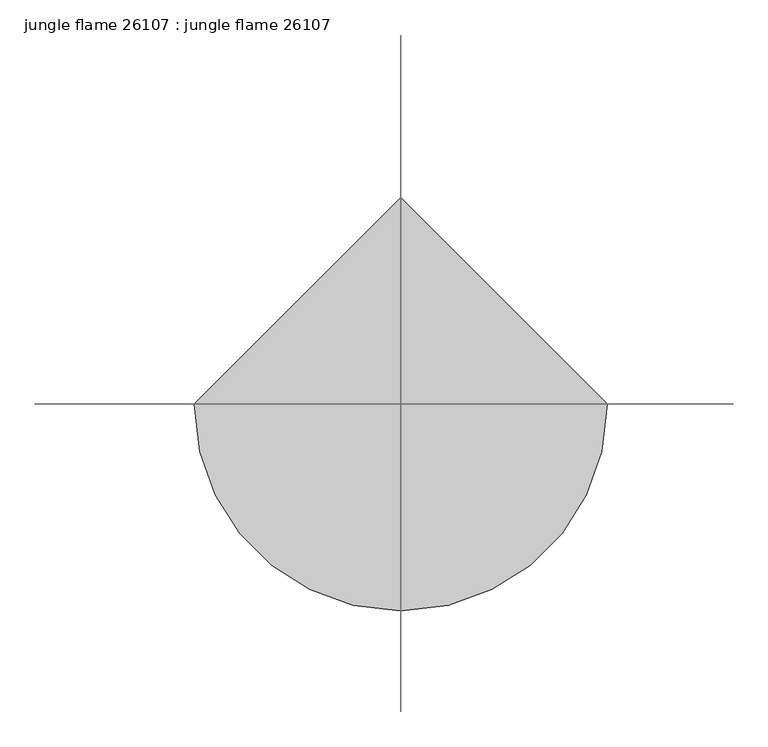
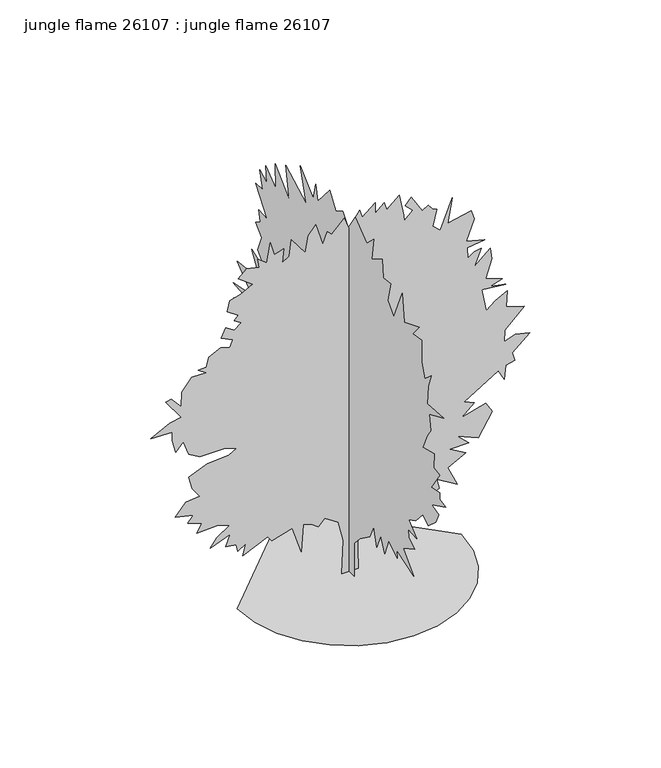
"""IFC4 building model written with IfcOpenShell, lengths in millimetres: proxy geometry, jungle flame 26107 : jungle flame 26107."""

import ifcopenshell
import ifcopenshell.guid

model = None  # the IFC model being written
_history = None  # IfcOwnerHistory: only IFC2X3 demands one
_inside = {}  # id of a spatial element -> (the spatial element, [elements in it])
_under = {}  # id of a project, library or spatial element -> (it, [spatial elements below it])
_declared = {}  # id of a project -> (the project, [libraries it declares])
_typed = {}  # id of a type object -> (the type object, [elements of that type])
_made_of = {}  # id of a material, layer set ... -> (it, [elements and type objects made of it])


def new_model(schema):
    """Start an empty IFC model of exactly this schema.

    Asked for "IFC4X3", IfcOpenShell would pick the latest addendum, in which some entities
    have other attributes; the version numbers below select the first issue.
    IFC2X3 requires an IfcOwnerHistory on every rooted entity: one is made here for all.
    """
    global model, _history
    if schema == "IFC4X3":
        model = ifcopenshell.file(schema_version=(4, 3, 0, 0))
    else:
        model = ifcopenshell.file(schema=schema)
    _inside.clear()
    _under.clear()
    _declared.clear()
    _typed.clear()
    _made_of.clear()
    _history = None
    if model.schema == "IFC2X3":
        org = make("IfcOrganization", Name="unknown")
        user = make(
            "IfcPersonAndOrganization",
            ThePerson=make("IfcPerson", FamilyName="unknown"),
            TheOrganization=org,
        )
        app = make(
            "IfcApplication",
            ApplicationDeveloper=org,
            Version="unknown",
            ApplicationFullName="unknown",
            ApplicationIdentifier="unknown",
        )
        _history = make(
            "IfcOwnerHistory",
            OwningUser=user,
            OwningApplication=app,
            ChangeAction="ADDED",
            CreationDate=0,
        )
    return model


def make(cls, **values):
    """One entity of the class cls with the attributes given. An attribute that is None is left unset."""
    return model.create_entity(
        cls, **{name: value for name, value in values.items() if value is not None}
    )


def rooted(cls, **values):
    """An entity with a GlobalId (a new one), such as an element, a storey or a relation."""
    return make(cls, GlobalId=ifcopenshell.guid.new(), OwnerHistory=_history, **values)


def si_unit(unit_type, name, prefix=None):
    """IfcSIUnit, for example si_unit("LENGTHUNIT", "METRE", prefix="MILLI")."""
    return make("IfcSIUnit", UnitType=unit_type, Prefix=prefix, Name=name)


def assignment(units):
    """IfcUnitAssignment: the units of a project."""
    return None if units is None else make("IfcUnitAssignment", Units=units)


def point(xyz):
    """IfcCartesianPoint."""
    return None if xyz is None else make("IfcCartesianPoint", Coordinates=xyz)


def direction(xyz):
    """IfcDirection."""
    return None if xyz is None else make("IfcDirection", DirectionRatios=xyz)


def frame(location, z_axis=None, x_axis=None):
    """IfcAxis2Placement3D, a coordinate frame: its origin and axes. An axis left out is left unset."""
    return make(
        "IfcAxis2Placement3D",
        Location=point(location),
        Axis=direction(z_axis),
        RefDirection=direction(x_axis),
    )


def origin():
    """The frame at (0, 0, 0) with its axes left unset."""
    return frame((0.0, 0.0, 0.0))


def place(relative_to, where):
    """IfcLocalPlacement: puts the frame where relative to a parent placement (None: the world)."""
    return make(
        "IfcLocalPlacement", PlacementRelTo=relative_to, RelativePlacement=where
    )


def context(
    kind, dimensions, precision=None, world=None, true_north=None, identifier=None
):
    """IfcGeometricRepresentationContext, for example the 3D "Model" context."""
    return make(
        "IfcGeometricRepresentationContext",
        ContextIdentifier=identifier,
        ContextType=kind,
        CoordinateSpaceDimension=dimensions,
        Precision=precision,
        WorldCoordinateSystem=world,
        TrueNorth=true_north,
    )


def project(units=None, contexts=None):
    """IfcProject with its units and contexts."""
    return rooted(
        "IfcProject",
        Name="project",
        RepresentationContexts=contexts,
        UnitsInContext=assignment(units),
    )


def spatial(cls, under=None, at=None, **own):
    """A site, building, storey or space (cls), placed at a placement, below another one or the project."""
    s = rooted(cls, ObjectPlacement=at, **own)
    if under is not None:
        _under.setdefault(under.id(), (under, []))[1].append(s)
    return s


def point_list(points):
    """IfcCartesianPointList2D or 3D."""
    cls = (
        "IfcCartesianPointList2D" if len(points[0]) == 2 else "IfcCartesianPointList3D"
    )
    return make(cls, CoordList=points)


def triangles(points, corners, closed=None, point_numbers=None):
    """IfcTriangulatedFaceSet: each triangle names its three corners, points numbered from 1."""
    return make(
        "IfcTriangulatedFaceSet",
        Coordinates=point_list(points),
        Closed=closed,
        CoordIndex=corners,
        PnIndex=point_numbers,
    )


def shape(context_of_items, identifier, shape_type, items):
    """IfcShapeRepresentation: the items that make up one representation, for example the "Body"."""
    return make(
        "IfcShapeRepresentation",
        ContextOfItems=context_of_items,
        RepresentationIdentifier=identifier,
        RepresentationType=shape_type,
        Items=items,
    )


def source(mapping_origin, context_of_items, identifier, shape_type, items):
    """IfcRepresentationMap: a shape defined once, which mapped items show again and again."""
    return make(
        "IfcRepresentationMap",
        MappingOrigin=mapping_origin,
        MappedRepresentation=shape(context_of_items, identifier, shape_type, items),
    )


def transform(
    local_origin,
    x_axis=None,
    y_axis=None,
    z_axis=None,
    scale=None,
    scale2=None,
    scale3=None,
    uniform=True,
):
    """IfcCartesianTransformationOperator3D, or its non-uniform kind. x_axis, y_axis, z_axis: its Axis1, 2, 3."""
    if uniform:
        return make(
            "IfcCartesianTransformationOperator3D",
            Axis1=direction(x_axis),
            Axis2=direction(y_axis),
            LocalOrigin=point(local_origin),
            Scale=scale,
            Axis3=direction(z_axis),
        )
    return make(
        "IfcCartesianTransformationOperator3DnonUniform",
        Axis1=direction(x_axis),
        Axis2=direction(y_axis),
        LocalOrigin=point(local_origin),
        Scale=scale,
        Axis3=direction(z_axis),
        Scale2=scale2,
        Scale3=scale3,
    )


def mapped(mapping_source, mapping_target):
    """IfcMappedItem: shows the shape of a source again, moved by a transform."""
    return make(
        "IfcMappedItem", MappingSource=mapping_source, MappingTarget=mapping_target
    )


def made_of(thing, what):
    """Note that an element or type object is made of a material, layer set ...; save() writes the relation."""
    if what is not None:
        _made_of.setdefault(what.id(), (what, []))[1].append(thing)
    return thing


def element(
    cls,
    number,
    at=None,
    inside=None,
    cuts=None,
    type_object=None,
    material=None,
    context=None,
    identifier="Body",
    shape_type=None,
    held_by="IfcProductDefinitionShape",
    body=None,
    shapes=None,
    **own,
):
    """One element of the class cls, such as IfcWall. Its Tag is "e" and its number.

    at: its placement. inside: the storey or other place that contains it. cuts: it is an
    opening in that element (IfcRelVoidsElement). A single representation is given by context,
    identifier, shape_type and body (its items); several are given by shapes. held_by: the class
    of the entity that holds the representations. save() writes the other relations.
    """
    e = rooted(cls, Tag="e%d" % number, ObjectPlacement=at, **own)
    if body is not None:
        shapes = [shape(context, identifier, shape_type, body)]
    if shapes is not None:
        e.Representation = make(held_by, Representations=shapes)
    if inside is not None:
        _inside.setdefault(inside.id(), (inside, []))[1].append(e)
    if cuts is not None:
        rooted(
            "IfcRelVoidsElement", RelatingBuildingElement=cuts, RelatedOpeningElement=e
        )
    if type_object is not None:
        _typed.setdefault(type_object.id(), (type_object, []))[1].append(e)
    return made_of(e, material)


def aggregate(whole, parts):
    """IfcRelAggregates: a whole, such as a stair, and the parts it consists of."""
    return rooted("IfcRelAggregates", RelatingObject=whole, RelatedObjects=parts)


def save(model, path):
    """Write the relations noted so far, then the file.

    IfcRelAggregates (storeys below a building ...), IfcRelContainedInSpatialStructure (elements
    in a storey), IfcRelDefinesByType, IfcRelAssociatesMaterial and IfcRelDeclares: one each for
    every whole, place, type object, material and project.
    """
    for whole, parts in _under.values():
        aggregate(whole, parts)
    for where, things in _inside.values():
        rooted(
            "IfcRelContainedInSpatialStructure",
            RelatedElements=things,
            RelatingStructure=where,
        )
    for kind, things in _typed.values():
        rooted("IfcRelDefinesByType", RelatedObjects=things, RelatingType=kind)
    for what, things in _made_of.values():
        rooted("IfcRelAssociatesMaterial", RelatedObjects=things, RelatingMaterial=what)
    for by, libraries in _declared.values():
        rooted("IfcRelDeclares", RelatingContext=by, RelatedDefinitions=libraries)
    model.write(path)


def jungle_flame_26107_jungle_flame_26107_31e44138(model_context):
    return source(origin(), model_context, "Body", "Tessellation", [
        triangles([(-297.8835799, 0.0, 5.16e-05), (-290.0095692, -68.2551316, 5.16e-05), (-267.5813779, -130.9367389, 5.16e-05), (-232.3950082, -186.2485517, 5.16e-05), (-186.2485517, -232.3952625, 5.16e-05), (-130.9367389, -267.5813779, 5.16e-05), (-68.2551316, -290.0095692, 5.16e-05), (1.3e-05, -297.8835799, 5.16e-05), (68.2551316, -290.0095692, 5.16e-05), (130.9367389, -267.5813779, 5.16e-05), (186.2485517, -232.3950082, 5.16e-05), (232.3952625, -186.2485517, 5.16e-05), (267.5813779, -130.9367389, 5.16e-05), (290.0095692, -68.2551316, 5.16e-05), (297.8835799, 2.6e-05, 5.16e-05), (-3.91e-05, 297.8835799, 5.16e-05), (-1.65e-05, -22.3446072, 4.98e-05), (-1.37e-05, -22.4089451, 93.4481205), (-1.4e-05, -48.2564431, 121.2837307), (-1.51e-05, -93.9863508, 155.0842657), (-1.48e-05, -113.868958, 194.849244), (-1.69e-05, -127.7866314, 145.1429666), (-1.64e-05, -145.6809334, 188.8845644), (-1.84e-05, -163.5752263, 149.1193318), (-1.77e-05, -181.4695374, 196.8375492), (-2.03e-05, -221.2347519, 170.9902534), (-1.95e-05, -219.2464467, 192.8611749), (-2.38e-05, -296.7888247, 167.0136247), (-2.02e-05, -249.070353, 216.7201655), (-2.16e-05, -300.7639273, 244.5557666), (-1.99e-05, -272.9306153, 260.4617543), (-1.92e-05, -270.9418014, 282.3336933), (-2.1e-05, -310.7054898, 280.3448793), (-1.85e-05, -274.9168858, 312.1558373), (-1.94e-05, -306.7304054, 328.0638416), (-1.98e-05, -338.5413634, 363.8524638), (-2.13e-05, -364.3884049, 349.9332553), (-2.2e-05, -398.1907022, 379.7579247), (-2.17e-05, -412.1073672, 409.5800869), (-2e-05, -380.2964092, 417.5353426), (-2.19e-05, -443.9208687, 449.3463006), (-2.05e-05, -416.0849951, 455.3102171), (-2e-05, -416.0849951, 473.2045464), (-1.85e-05, -378.3075771, 465.2517978), (-1.85e-05, -416.0849951, 522.9123407), (-1.71e-05, -388.2491578, 526.8874251), (-1.6e-05, -390.2379536, 566.6536752), (-1.41e-05, -338.5413634, 554.7232987), (-1.37e-05, -358.4244884, 598.4646332), (-1.37e-05, -374.3299493, 622.325386), (-1.22e-05, -368.3660328, 664.0779247), (-1.42e-05, -433.9793243, 693.9025578), (-1.1e-05, -358.4244884, 687.9386776), (-9.7e-06, -364.3884049, 741.6215927), (-9.1e-06, -376.3187814, 777.4101786), (-8.6e-06, -346.4940757, 751.5605936), (-6.8e-06, -332.5774469, 789.3380116), (-5e-06, -332.5774469, 850.9736389), (-3.4e-06, -292.8111969, 845.0096861), (-3.7e-06, -322.6358663, 880.7983446), (-1.4e-06, -253.0469816, 852.962471), (1.3e-06, -243.1056735, 928.5173069), (3e-07, -205.3287642, 839.0458059), (2.5e-06, -177.4931631, 868.8679682), (3.5e-06, -191.4108456, 924.5396427), (4.9e-06, -157.6105468, 920.564522), (6.6e-06, -151.6456129, 968.2810135), (7.9e-06, -103.9276498, 940.4451399), (9.3e-06, -111.8806437, 1000.0944786), (9.9e-06, -80.0684139, 970.2698456), (1.34e-05, -28.3738313, 1012.0223116), (1.33e-05, 3.4383978, 962.3170607), (1.55e-05, 29.285692, 994.128055), (1.63e-05, 61.0979195, 976.2337257), (1.88e-05, 88.9335251, 1015.9999758), (1.94e-05, 144.6047364, 952.3755163), (2.1e-05, 154.5460354, 994.128055), (2.02e-05, 166.475667, 946.4115635), (2.45e-05, 226.1232435, 1002.0833107), (2.06e-05, 198.2876424, 912.6118097), (2.63e-05, 291.7367712, 964.3058928), (2.3e-05, 275.8287488, 876.8232239), (2.77e-05, 339.4532264, 938.4588512), (2.56e-05, 337.4669377, 870.8567276), (2.87e-05, 383.1945608, 906.6453861), (2.71e-05, 379.2194401, 860.9151833), (2.91e-05, 411.0303981, 878.8095125), (2.7e-05, 397.113733, 831.0930937), (2.85e-05, 430.9135231, 829.1042616), (2.4e-05, 377.2306443, 759.5158493), (2.58e-05, 415.0080623, 763.49097), (2.47e-05, 409.0441458, 733.6662643), (2.52e-05, 430.9135231, 719.7495993), (2.32e-05, 403.0776858, 691.9137983), (2.26e-05, 420.9719788, 648.1724276), (1.97e-05, 381.2082722, 608.4061775), (2.34e-05, 448.807816, 632.2669304), (1.9e-05, 401.0888537, 554.7232987), (2.1e-05, 436.8774396, 568.6424709), (2.42e-05, 514.4211076, 558.7009266), (1.96e-05, 448.807816, 505.0180115), (2.28e-05, 532.3154005, 487.1237185), (1.85e-05, 440.8551038, 479.1710063), (1.74e-05, 430.9135231, 457.2990492), (2.16e-05, 530.3266047, 447.3575048), (1.66e-05, 438.8662717, 419.5216312), (1.6e-05, 456.7605646, 369.8163803), (1.51e-05, 409.0441458, 411.5688827), (1.33e-05, 395.1249372, 371.8051761), (1.47e-05, 442.8438995, 349.9332553), (1.34e-05, 444.8327316, 302.2142748), (9.7e-06, 379.2194401, 276.3672333), (1.12e-05, 426.9384387, 254.4978378), (5.4e-06, 323.5477292, 216.7201655), (7.3e-06, 379.2194401, 194.849244), (7.4e-06, 411.0303981, 151.1076461), (4.7e-06, 327.5253571, 184.9081902), (2.9e-06, 321.5588971, 135.2016584), (2.6e-06, 287.7591252, 174.966882), (0.0, 265.8897297, 119.2956707), (1.8e-06, 267.8760183, 176.9549329), (1.3e-06, 253.9588446, 182.9198668), (-1.2e-06, 226.1232435, 141.1663379), (-2e-07, 228.1115487, 170.9902534), (-2.1e-06, 180.3933313, 176.9549329), (-2.7e-06, 186.3580108, 151.1076461), (-3.4e-06, 154.5460354, 174.966882), (-6.1e-06, 144.6047364, 99.4130544), (-6.1e-06, 82.9688456, 190.8728697), (-7.1e-06, 69.0509133, 178.9432563), (-8.2e-06, 41.2153077, 182.9198668), (-8.5e-06, 57.1215497, 149.1193318), (-9.5e-06, 17.3562001, 174.966882), (-1.44e-05, 25.309295, 5.13e-05), (-19.2607679, 5.89e-05, 1.9e-06), (-15.3064967, 5.32e-05, 92.9241154), (-29.1462451, 5.05e-05, 148.2829094), (-64.7341846, 5.06e-05, 172.0082871), (-82.5281566, 5.25e-05, 154.2143151), (-100.3221195, 5.24e-05, 168.0540227), (-122.0703651, 5.3e-05, 173.9854194), (-128.0015165, 5.76e-05, 100.8324082), (-151.7268943, 5.43e-05, 173.9854194), (-205.1088103, 5.76e-05, 158.1685977), (-216.9713675, 5.72e-05, 173.9854194), (-282.2168581, 6.19e-05, 142.351758), (-274.3072937, 5.97e-05, 173.9854194), (-296.0547671, 6.15e-05, 160.14573), (-300.0095584, 6.05e-05, 179.9165799), (-327.6904633, 6.14e-05, 183.8708443), (-315.8261438, 5.9e-05, 215.5045239), (-369.2092953, 6.27e-05, 193.7565236), (-351.4140879, 6.05e-05, 217.4816561), (-317.8048021, 5.76e-05, 241.2070248), (-351.4140879, 5.85e-05, 251.0924498), (-404.7972393, 6.09e-05, 249.1153175), (-390.956805, 5.9e-05, 270.8630453), (-428.5208639, 5.98e-05, 284.7035159), (-414.6829368, 5.82e-05, 302.4962162), (-462.1326568, 5.95e-05, 314.3605356), (-434.4542953, 5.64e-05, 345.9937065), (-396.887693, 5.46e-05, 349.9484797), (-416.6590516, 5.38e-05, 377.6268774), (-426.5447127, 5.21e-05, 413.2148214), (-377.1163344, 4.86e-05, 434.9622949), (-319.780917, 4.59e-05, 438.917068), (-298.0334254, 4.42e-05, 450.7814238), (-333.6213876, 4.52e-05, 460.6645414), (-396.887693, 4.8e-05, 460.6645414), (-426.5447127, 4.82e-05, 478.4597852), (-440.3851833, 4.64e-05, 518.0025023), (-460.1565419, 4.86e-05, 496.2524855), (-470.0396959, 4.69e-05, 531.8404295), (-470.0396959, 4.55e-05, 555.5665612), (-527.3776568, 4.79e-05, 557.5426761), (-475.9731274, 4.41e-05, 583.2475024), (-446.3160713, 4.25e-05, 589.1783904), (-487.8349397, 4.09e-05, 646.5138079), (-472.0183542, 4e-05, 648.4899227), (-446.3160713, 4.07e-05, 618.8354101), (-444.337413, 3.82e-05, 658.3755838), (-418.6351665, 3.51e-05, 691.987413), (-379.0949927, 3.35e-05, 690.0087547), (-400.8424662, 3.35e-05, 705.8278473), (-379.0949927, 3.26e-05, 705.8278473), (-373.1615613, 3.08e-05, 731.5301302), (-341.5283904, 2.84e-05, 747.346752), (-317.8048021, 2.79e-05, 739.437133), (-309.8952195, 2.64e-05, 759.2085279), (-339.5522756, 2.68e-05, 773.0489622), (-327.6904633, 2.48e-05, 798.7512451), (-305.9404464, 2.47e-05, 784.9108109), (-286.1690878, 2.3e-05, 798.7512451), (-305.9404464, 2.31e-05, 810.6130211), (-294.0786522, 2.19e-05, 822.4748697), (-323.7356901, 2.2e-05, 842.246192), (-317.8048021, 2e-05, 871.903248), (-288.1477461, 1.82e-05, 879.8127943), (-256.5145934, 1.59e-05, 895.6293434), (-294.0786522, 1.58e-05, 925.2863995), (-272.3311788, 1.36e-05, 945.0577944), (-238.719604, 1.26e-05, 937.1482481), (-242.6736322, 1.14e-05, 960.8743435), (-218.9484997, 1.14e-05, 943.0791361), (-209.0628204, 7.8e-06, 996.4622875), (-199.1773955, 9.6e-06, 958.8956852), (-173.4748764, 8e-06, 966.8052315), (-177.429159, 1.04e-05, 929.2386292), (-159.635187, 8.9e-06, 941.1030212), (-153.7037722, 6.1e-06, 984.5979681), (-116.1389593, 7.4e-06, 935.1721333), (-108.2304123, 4.3e-06, 980.6457384), (-88.459308, 2.1e-06, 1004.3692904), (-70.6655904, 4.9e-06, 943.0791361), (-58.8027788, 2.5e-06, 974.712307), (-46.9402171, 2.7e-06, 962.8504583), (-13.329386, -7e-07, 996.4622875), (-1.4667204, 6e-07, 964.8265732), (28.1899354, -3e-06, 1004.3692904), (34.1210891, -2e-06, 982.6218533), (69.7090263, -5.2e-06, 1010.300251), (69.7090263, -3.4e-06, 980.6457384), (93.4344041, -5.8e-06, 1002.3931755), (99.3655555, -4.7e-06, 980.6457384), (132.9763673, -8e-06, 1010.300251), (144.8391788, -4.8e-06, 949.0100241), (146.816311, -4e-06, 933.1934023), (168.5642931, -6.2e-06, 954.9434555), (148.793198, -6.5e-06, 974.712307), (164.610283, -8.3e-06, 992.5075144), (194.2668122, -6.8e-06, 945.0577944), (210.083652, -8e-06, 954.9434555), (219.969077, -7.6e-06, 941.1030212), (231.8318885, -7.8e-06, 935.1721333), (221.9462092, -4.8e-06, 891.6745703), (241.7173134, -4.6e-06, 873.8819063), (273.3497213, -1.07e-05, 952.9647972), (261.487909, -6.2e-06, 885.7436823), (324.756776, -9.8e-06, 899.5841892), (332.6637789, -8.6e-06, 873.8819063), (310.9163054, -4.3e-06, 818.5225674), (360.3447201, -5.7e-06, 804.6821331), (312.8924203, -3.2e-06, 798.7512451), (314.8710786, -1.5e-06, 769.0941891), (332.6637789, -3e-06, 780.9560377), (350.4590226, -4e-06, 784.9108109), (332.6637789, -6e-07, 739.437133), (374.1826472, -4.6e-06, 777.0037354), (378.1374204, -2.9e-06, 745.3680937), (362.3208349, 7e-07, 695.9421862), (405.8183252, -2e-07, 680.1256371), (374.1826472, 1.8e-06, 670.2399759), (415.7014792, 5e-07, 660.3542421), (352.4351375, 2.8e-06, 668.2613176), (364.2969498, 6.1e-06, 604.9949759), (388.0230815, 3.9e-06, 624.7662981), (419.6562524, 1.5e-06, 640.5829199), (417.6801375, 4.2e-06, 597.0853932), (465.1298575, 3.1e-06, 581.2688441), (413.7253644, 8.3e-06, 531.8404295), (411.7492132, 1.02e-05, 500.2072586), (441.4037258, 8.2e-06, 512.0716144), (478.9703281, 7.2e-06, 502.1859169), (433.496723, 1.15e-05, 462.6431997), (439.427611, 1.27e-05, 438.917068), (415.7014792, 1.41e-05, 432.98618), (411.7492132, 1.65e-05, 395.4221211), (395.9326641, 1.54e-05, 425.0765974), (304.9854175, 2.27e-05, 369.7198382), (332.6637789, 2.22e-05, 357.8555188), (297.075853, 2.55e-05, 328.1984628), (362.3208349, 2.16e-05, 345.9937065), (380.1135352, 2.26e-05, 316.3366868), (342.5494763, 2.79e-05, 255.046478), (287.1901737, 2.89e-05, 278.7726098), (316.8472298, 2.92e-05, 251.0924498), (267.4188151, 3.15e-05, 249.1153175), (308.9376472, 3.11e-05, 225.3902032), (261.487909, 3.47e-05, 199.6876841), (287.1901737, 3.69e-05, 144.3286358), (231.8316341, 3.73e-05, 177.9394476), (239.7401812, 3.86e-05, 150.2600507), (200.1979727, 4.14e-05, 132.4660787), (162.6331508, 4.11e-05, 166.0768723), (168.5642931, 4.56e-05, 85.0155775), (146.816311, 4.22e-05, 158.1685977), (91.4572718, 4.73e-05, 112.6949744), (101.3426968, 4.41e-05, 160.14573), (59.8236013, 4.92e-05, 104.7866817), (47.9607853, 4.76e-05, 140.3746166), (73.6632998, 4.26e-05, 205.6190989), (38.0753603, 4.45e-05, 199.6876841), (20.2813656, 4.7e-05, 170.0311549), (24.2355619, 5.7e-05, 0.0)], [[15, 16, 1], [14, 15, 1], [14, 1, 2], [13, 14, 2], [13, 2, 3], [13, 3, 4], [12, 13, 4], [11, 12, 4], [11, 4, 5], [11, 5, 6], [11, 6, 7], [11, 7, 8], [11, 8, 9], [11, 9, 10], [101, 102, 103], [119, 120, 121], [51, 52, 53], [104, 105, 106], [76, 77, 78], [27, 28, 29], [59, 60, 61], [106, 107, 108], [78, 79, 80], [122, 123, 124], [61, 62, 63], [54, 55, 56], [131, 132, 133], [115, 116, 117], [114, 115, 117], [21, 22, 23], [40, 41, 42], [32, 33, 34], [96, 97, 98], [68, 69, 70], [125, 126, 127], [127, 128, 129], [82, 83, 84], [86, 87, 88], [112, 113, 114], [23, 24, 25], [99, 100, 101], [84, 85, 86], [117, 118, 119], [80, 81, 82], [25, 26, 27], [88, 89, 90], [29, 30, 31], [44, 45, 46], [66, 67, 68], [64, 65, 66], [90, 91, 92], [46, 47, 48], [74, 75, 76], [92, 93, 94], [42, 43, 44], [40, 42, 44], [38, 39, 40], [98, 99, 101], [57, 58, 59], [70, 71, 72], [133, 134, 17], [133, 17, 18], [133, 18, 19], [104, 106, 108], [114, 117, 119], [72, 73, 74], [133, 19, 20], [37, 38, 40], [36, 37, 40], [133, 20, 21], [110, 111, 112], [109, 110, 112], [44, 46, 48], [53, 54, 56], [94, 95, 96], [98, 101, 103], [90, 92, 94], [68, 70, 72], [114, 119, 121], [114, 121, 122], [98, 103, 104], [129, 130, 131], [64, 66, 68], [86, 88, 90], [84, 86, 90], [82, 84, 90], [25, 27, 29], [25, 29, 31], [25, 31, 32], [57, 59, 61], [57, 61, 63], [56, 57, 63], [53, 56, 63], [98, 104, 108], [49, 50, 51], [36, 40, 44], [36, 44, 48], [35, 36, 48], [34, 35, 48], [25, 32, 34], [23, 25, 34], [21, 23, 34], [21, 34, 48], [133, 21, 48], [131, 133, 48], [129, 131, 48], [90, 94, 96], [82, 90, 96], [80, 82, 96], [109, 112, 114], [109, 114, 122], [64, 68, 72], [122, 124, 125], [109, 122, 125], [109, 125, 127], [109, 127, 129], [109, 129, 48], [108, 109, 48], [98, 108, 48], [96, 98, 48], [80, 96, 48], [78, 80, 48], [76, 78, 48], [74, 76, 48], [72, 74, 48], [64, 72, 48], [63, 64, 48], [53, 63, 48], [53, 48, 49], [53, 49, 51], [252, 253, 254], [236, 237, 238], [284, 285, 286], [141, 142, 143], [241, 242, 243], [204, 205, 206], [174, 175, 176], [151, 152, 153], [279, 280, 281], [266, 267, 268], [183, 184, 185], [250, 251, 252], [151, 153, 154], [286, 287, 288], [202, 203, 204], [209, 210, 211], [275, 276, 277], [145, 146, 147], [218, 219, 220], [220, 221, 222], [247, 248, 249], [288, 289, 290], [288, 290, 291], [155, 156, 157], [262, 263, 264], [212, 213, 214], [211, 212, 214], [245, 246, 247], [244, 245, 247], [171, 172, 173], [277, 278, 279], [261, 262, 264], [224, 225, 226], [256, 257, 258], [177, 178, 179], [177, 179, 180], [258, 259, 260], [222, 223, 224], [159, 160, 161], [269, 270, 271], [247, 249, 250], [216, 217, 218], [214, 215, 216], [206, 207, 208], [147, 148, 149], [250, 252, 254], [159, 161, 162], [157, 158, 159], [229, 230, 231], [228, 229, 231], [193, 194, 195], [149, 150, 151], [199, 200, 201], [199, 201, 202], [190, 191, 192], [189, 190, 192], [294, 135, 136], [293, 294, 136], [293, 136, 137], [204, 206, 208], [174, 176, 177], [264, 265, 266], [231, 232, 233], [238, 239, 240], [238, 240, 241], [236, 238, 241], [138, 139, 140], [255, 256, 258], [255, 258, 260], [163, 164, 165], [281, 282, 283], [281, 283, 284], [273, 274, 275], [272, 273, 275], [271, 272, 275], [233, 234, 235], [231, 233, 235], [162, 163, 165], [162, 165, 166], [143, 144, 145], [195, 196, 197], [195, 197, 198], [227, 228, 231], [227, 231, 235], [171, 173, 174], [171, 174, 177], [261, 264, 266], [261, 266, 268], [195, 198, 199], [293, 137, 138], [292, 293, 138], [157, 159, 162], [155, 157, 162], [155, 162, 166], [154, 155, 166], [154, 166, 167], [286, 288, 291], [284, 286, 291], [181, 182, 183], [180, 181, 183], [247, 250, 254], [147, 149, 151], [185, 186, 187], [185, 187, 188], [183, 185, 188], [199, 202, 204], [199, 204, 208], [224, 226, 227], [277, 279, 281], [277, 281, 284], [277, 284, 291], [261, 268, 269], [189, 192, 193], [236, 241, 243], [193, 195, 199], [193, 199, 208], [145, 147, 151], [145, 151, 154], [145, 154, 167], [143, 145, 167], [141, 143, 167], [222, 224, 227], [275, 277, 291], [271, 275, 291], [269, 271, 291], [177, 180, 183], [140, 141, 167], [138, 140, 167], [292, 138, 167], [291, 292, 167], [269, 291, 167], [261, 269, 167], [260, 261, 167], [255, 260, 167], [254, 255, 167], [247, 254, 167], [244, 247, 167], [243, 244, 167], [236, 243, 167], [235, 236, 167], [227, 235, 167], [222, 227, 167], [220, 222, 167], [218, 220, 167], [216, 218, 167], [214, 216, 167], [211, 214, 167], [209, 211, 167], [208, 209, 167], [193, 208, 167], [189, 193, 167], [188, 189, 167], [183, 188, 167], [177, 183, 167], [177, 167, 168], [171, 177, 168], [171, 168, 169], [170, 171, 169]], closed=False),
    ])


if __name__ == "__main__":
    model = new_model("IFC4")
    model_context = context("Model", 3, world=origin())
    ifc_project = project(units=[si_unit("LENGTHUNIT", "METRE", prefix="MILLI")], contexts=[model_context])
    site = spatial("IfcSite", under=ifc_project)
    building = spatial("IfcBuilding", under=site)
    placement = place(None, origin())
    jungle_flame_26107_jungle_flame_26107_shape = jungle_flame_26107_jungle_flame_26107_31e44138(model_context)
    element("IfcBuildingElementProxy", 1, Name="jungle flame 26107 : jungle flame 26107", ObjectType="jungle flame 26107 : jungle flame 26107", at=placement, inside=building, context=model_context, shape_type="MappedRepresentation", body=[
        mapped(jungle_flame_26107_jungle_flame_26107_shape, transform((0.0, 0.0, 0.0), x_axis=(1.0, 0.0, 0.0), y_axis=(0.0, 1.0, 0.0), z_axis=(0.0, 0.0, 1.0))),
    ])
    save(model, "model.ifc")

# Revit data of these elements
# Type "jungle flame 26107 : jungle flame 26107"
#   built-in parameter 1005195 = "RPC-16-FUVJ-JWG0-MWGK-8000-ST1L-LVER-AU"
#   Height = 0
